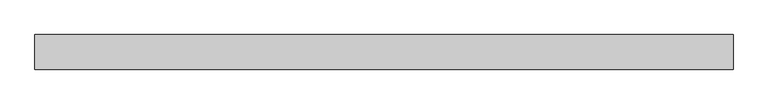
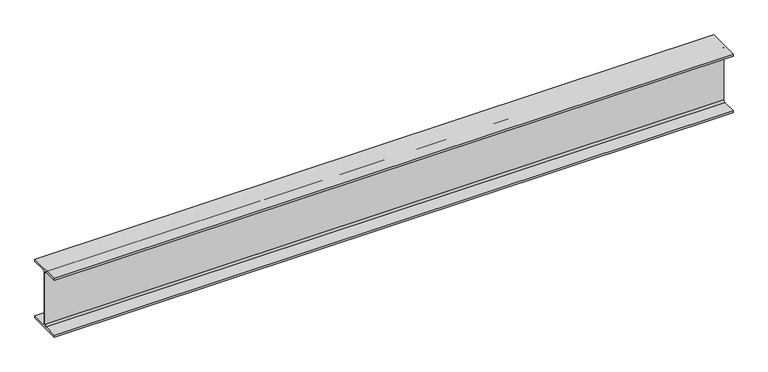
"""IFC4 building model written with IfcOpenShell, lengths in millimetres: beam geometry, Old_Steel Beam_H-KSD3502 : H_SB_ASB_H-200×200x8x12."""

from ifc_helpers import new_model, si_unit, point, frame, frame_2d, origin, place, context, project, spatial, polyline, circle_curve, trimmed, segment, composite_curve, outline, extrude, source, transform, mapped, element, save


def beam_fe0ad751(model_context):
    return source(origin(), model_context, "Body", "SweptSolid", [
        extrude(outline(composite_curve([segment(polyline([(82.5, -141.5), (82.5, -151.7), (-82.5, -151.7), (-82.5, -141.5), (-11.9, -141.5)]), True, "CONTINUOUS"), segment(trimmed(circle_curve(frame_2d((-11.9, -132.6)), 8.9), [point((-11.9, -141.5))], [point((-3.0, -132.6))], True, "CARTESIAN"), True, "CONTINUOUS"), segment(polyline([(-3.0, -132.6), (-3.0, 132.6)]), True, "CONTINUOUS"), segment(trimmed(circle_curve(frame_2d((-11.9, 132.6)), 8.9), [point((-3.0, 132.6))], [point((-11.9, 141.5))], True, "CARTESIAN"), True, "CONTINUOUS"), segment(polyline([(-11.9, 141.5), (-82.5, 141.5), (-82.5, 151.7), (82.5, 151.7), (82.5, 141.5), (11.9, 141.5)]), True, "CONTINUOUS"), segment(trimmed(circle_curve(frame_2d((11.9, 132.6)), 8.9), [point((11.9, 141.5))], [point((3.0, 132.6))], True, "CARTESIAN"), True, "CONTINUOUS"), segment(polyline([(3.0, 132.6), (3.0, -132.6)]), True, "CONTINUOUS"), segment(trimmed(circle_curve(frame_2d((11.9, -132.6)), 8.9), [point((3.0, -132.6))], [point((11.9, -141.5))], True, "CARTESIAN"), True, "CONTINUOUS"), segment(polyline([(11.9, -141.5), (82.5, -141.5)]), True, "CONTINUOUS")], self_intersect=False)), frame((-1716.7775834, 0.0, 0.0), z_axis=(1.0, 0.0, 0.0), x_axis=(0.0, 1.0, 0.0)), (0.0, 0.0, 1.0), 3324.8852978),
    ])


if __name__ == "__main__":
    model = new_model("IFC4")
    model_context = context("Model", 3, world=origin())
    ifc_project = project(units=[si_unit("LENGTHUNIT", "METRE", prefix="MILLI")], contexts=[model_context])
    site = spatial("IfcSite", under=ifc_project)
    building = spatial("IfcBuilding", under=site)
    placement = place(None, origin())
    beam_shape = beam_fe0ad751(model_context)
    element("IfcBeam", 1, ObjectType="Old_Steel Beam_H-KSD3502 : H_SB_ASB_H-200×200x8x12", at=placement, inside=building, context=model_context, shape_type="MappedRepresentation", body=[
        mapped(beam_shape, transform((0.0, 0.0, 0.0), x_axis=(1.0, 0.0, 0.0), y_axis=(0.0, 1.0, 0.0), z_axis=(0.0, 0.0, 1.0))),
    ])
    save(model, "model.ifc")

# Revit data of these elements
# Type "Old_Steel Beam_H-KSD3502 : H_SB_ASB_H-200×200x8x12"
#   Width = 20.0 cm
#   Web Thickness = 0.8 cm
#   Web Fillet = 1.3 cm
#   Warping Constant = 141376.0 cm⁶
#   Torsional Moment of Inertia = 26.2485 cm⁴
#   Torsional Modulus = 1.0 cm³
#   Section Area = 63.53 cm²
#   Plastic Modulus weak axis = 244.0 cm³
#   Plastic Modulus strong axis = 525.0 cm³
#   Perimeter = 1.16 m²/m
#   Nominal Weight = 49.90 kgf/m
#   Moment of Inertia weak axis = 1600.00 cm⁴
#   Moment of Inertia strong axis = 4720.00 cm⁴
#   Height = 20.0 cm
#   Flange Thickness = 1.2 cm
#   Elastic Modulus weak axis = 160.0 cm³
#   Elastic Modulus strong axis = 472.0 cm³
#   Centroid Vertical = 10.0 cm
#   Centroid Horizontal = 10.0 cm
#   Length [instance default] = 1.5240 m
#   Structural Material [instance default] = Steel, 45-345
#   Assembly Code = ""
# Element 1 (IfcBeam, "Old_Steel Beam_H-KSD3502 : H_SB_ASB_H-200×200x8x12")
#   Structural Material = none
# Materials
#   "Steel, 45-345": class "Metal", colour RGB 189 187 185, transparency 0, Description = "Steel 345 MPa", Cost = 0
